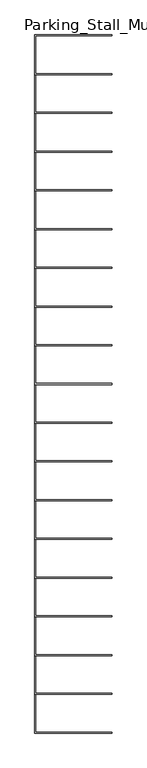
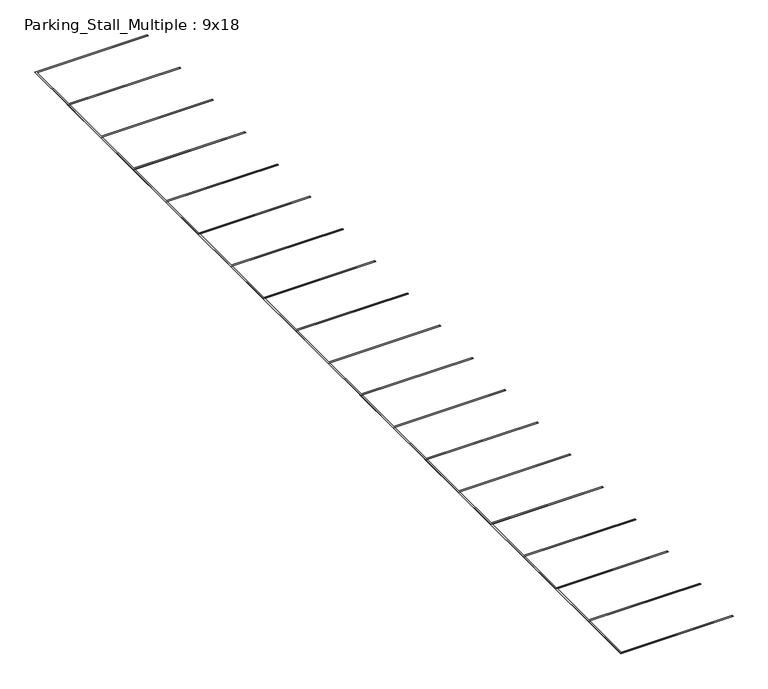
"""IFC4 building model written with IfcOpenShell, lengths in millimetres: proxy geometry, Parking_Stall_Multiple : 9x18."""

from ifc_helpers import new_model, si_unit, origin, origin_with_axes, place, context, project, spatial, polyline, outline, extrude, source, transform, mapped, element, save


def parking_stall_multiple_9x18_6e9e5a27(model_context):
    return source(origin(), model_context, "Body", "SweptSolid", [
        extrude(outline(polyline([(5486.4, 46634.4), (0.0, 46634.4), (0.0, 49453.8), (5486.4, 49453.8), (5486.4, 49377.6), (76.2, 49377.6), (76.2, 46710.6), (5486.4, 46710.6), (5486.4, 46634.4)])), origin_with_axes(), (0.0, 0.0, 1.0), 6.35),
        extrude(outline(polyline([(5486.4, 43891.2), (0.0, 43891.2), (0.0, 46710.6), (5486.4, 46710.6), (5486.4, 46634.4), (76.2, 46634.4), (76.2, 43967.4), (5486.4, 43967.4), (5486.4, 43891.2)])), origin_with_axes(), (0.0, 0.0, 1.0), 6.35),
        extrude(outline(polyline([(5486.4, 41148.0), (0.0, 41148.0), (0.0, 43967.4), (5486.4, 43967.4), (5486.4, 43891.2), (76.2, 43891.2), (76.2, 41224.2), (5486.4, 41224.2), (5486.4, 41148.0)])), origin_with_axes(), (0.0, 0.0, 1.0), 6.35),
        extrude(outline(polyline([(5486.4, 38404.8), (0.0, 38404.8), (0.0, 41224.2), (5486.4, 41224.2), (5486.4, 41148.0), (76.2, 41148.0), (76.2, 38481.0), (5486.4, 38481.0), (5486.4, 38404.8)])), origin_with_axes(), (0.0, 0.0, 1.0), 6.35),
        extrude(outline(polyline([(5486.4, 35661.6), (0.0, 35661.6), (0.0, 38481.0), (5486.4, 38481.0), (5486.4, 38404.8), (76.2, 38404.8), (76.2, 35737.8), (5486.4, 35737.8), (5486.4, 35661.6)])), origin_with_axes(), (0.0, 0.0, 1.0), 6.35),
        extrude(outline(polyline([(5486.4, 32918.4), (0.0, 32918.4), (0.0, 35737.8), (5486.4, 35737.8), (5486.4, 35661.6), (76.2, 35661.6), (76.2, 32994.6), (5486.4, 32994.6), (5486.4, 32918.4)])), origin_with_axes(), (0.0, 0.0, 1.0), 6.35),
        extrude(outline(polyline([(5486.4, 30175.2), (0.0, 30175.2), (0.0, 32994.6), (5486.4, 32994.6), (5486.4, 32918.4), (76.2, 32918.4), (76.2, 30251.4), (5486.4, 30251.4), (5486.4, 30175.2)])), origin_with_axes(), (0.0, 0.0, 1.0), 6.35),
        extrude(outline(polyline([(5486.4, 27432.0), (0.0, 27432.0), (0.0, 30251.4), (5486.4, 30251.4), (5486.4, 30175.2), (76.2, 30175.2), (76.2, 27508.2), (5486.4, 27508.2), (5486.4, 27432.0)])), origin_with_axes(), (0.0, 0.0, 1.0), 6.35),
        extrude(outline(polyline([(5486.4, 24688.8), (0.0, 24688.8), (0.0, 27508.2), (5486.4, 27508.2), (5486.4, 27432.0), (76.2, 27432.0), (76.2, 24765.0), (5486.4, 24765.0), (5486.4, 24688.8)])), origin_with_axes(), (0.0, 0.0, 1.0), 6.35),
        extrude(outline(polyline([(5486.4, 21945.6), (0.0, 21945.6), (0.0, 24765.0), (5486.4, 24765.0), (5486.4, 24688.8), (76.2, 24688.8), (76.2, 22021.8), (5486.4, 22021.8), (5486.4, 21945.6)])), origin_with_axes(), (0.0, 0.0, 1.0), 6.35),
        extrude(outline(polyline([(5486.4, 19202.4), (0.0, 19202.4), (0.0, 22021.8), (5486.4, 22021.8), (5486.4, 21945.6), (76.2, 21945.6), (76.2, 19278.6), (5486.4, 19278.6), (5486.4, 19202.4)])), origin_with_axes(), (0.0, 0.0, 1.0), 6.35),
        extrude(outline(polyline([(5486.4, 16459.2), (0.0, 16459.2), (0.0, 19278.6), (5486.4, 19278.6), (5486.4, 19202.4), (76.2, 19202.4), (76.2, 16535.4), (5486.4, 16535.4), (5486.4, 16459.2)])), origin_with_axes(), (0.0, 0.0, 1.0), 6.35),
        extrude(outline(polyline([(5486.4, 13716.0), (0.0, 13716.0), (0.0, 16535.4), (5486.4, 16535.4), (5486.4, 16459.2), (76.2, 16459.2), (76.2, 13792.2), (5486.4, 13792.2), (5486.4, 13716.0)])), origin_with_axes(), (0.0, 0.0, 1.0), 6.35),
        extrude(outline(polyline([(5486.4, 10972.8), (0.0, 10972.8), (0.0, 13792.2), (5486.4, 13792.2), (5486.4, 13716.0), (76.2, 13716.0), (76.2, 11049.0), (5486.4, 11049.0), (5486.4, 10972.8)])), origin_with_axes(), (0.0, 0.0, 1.0), 6.35),
        extrude(outline(polyline([(5486.4, 8229.6), (0.0, 8229.6), (0.0, 11049.0), (5486.4, 11049.0), (5486.4, 10972.8), (76.2, 10972.8), (76.2, 8305.8), (5486.4, 8305.8), (5486.4, 8229.6)])), origin_with_axes(), (0.0, 0.0, 1.0), 6.35),
        extrude(outline(polyline([(5486.4, 5486.4), (0.0, 5486.4), (0.0, 8305.8), (5486.4, 8305.8), (5486.4, 8229.6), (76.2, 8229.6), (76.2, 5562.6), (5486.4, 5562.6), (5486.4, 5486.4)])), origin_with_axes(), (0.0, 0.0, 1.0), 6.35),
        extrude(outline(polyline([(5486.4, 2743.2), (0.0, 2743.2), (0.0, 5562.6), (5486.4, 5562.6), (5486.4, 5486.4), (76.2, 5486.4), (76.2, 2819.4), (5486.4, 2819.4), (5486.4, 2743.2)])), origin_with_axes(), (0.0, 0.0, 1.0), 6.35),
        extrude(outline(polyline([(5486.4, 0.0), (0.0, 0.0), (0.0, 2819.4), (5486.4, 2819.4), (5486.4, 2743.2), (76.2, 2743.2), (76.2, 76.2), (5486.4, 76.2), (5486.4, 0.0)])), origin_with_axes(), (0.0, 0.0, 1.0), 6.35),
    ])


if __name__ == "__main__":
    model = new_model("IFC4")
    model_context = context("Model", 3, world=origin())
    ifc_project = project(units=[si_unit("LENGTHUNIT", "METRE", prefix="MILLI")], contexts=[model_context])
    site = spatial("IfcSite", under=ifc_project)
    building = spatial("IfcBuilding", under=site)
    placement = place(None, origin())
    parking_stall_multiple_9x18_shape = parking_stall_multiple_9x18_6e9e5a27(model_context)
    element("IfcBuildingElementProxy", 1, Name="Parking_Stall_Multiple : 9x18", ObjectType="Parking_Stall_Multiple : 9x18", at=placement, inside=building, context=model_context, shape_type="MappedRepresentation", body=[
        mapped(parking_stall_multiple_9x18_shape, transform((0.0, 0.0, 0.0), x_axis=(1.0, 0.0, 0.0), y_axis=(0.0, 1.0, 0.0), z_axis=(0.0, 0.0, 1.0))),
    ])
    save(model, "model.ifc")

# Revit data of these elements
# Type "Parking_Stall_Multiple : 9x18"
#   Type Mark = "PK-1"
#   Parking_Width_M = 9' - 0"
#   Parking_Run_Length [instance default] = 65' - 0"
#   Parking_Line_Width = 0' - 3"
#   Parking_Length_M = 18' - 0"
#   Single_Parking_Visibility [instance default] = no
#   Parking_ADA_Symbol = no
#   ParkingUnitsArray [instance default] = 7
#   ParkingUnits [instance default] = 7
#   Multiple_Parking_Visibility [instance default] = yes
#   Parking_Line_Material = none
# Element 1 (IfcBuildingElementProxy, "Parking_Stall_Multiple : 9x18")
#   Parking_Run_Length = 160' - 6"
#   ParkingUnitsArray = 18
#   ParkingUnits = 18
